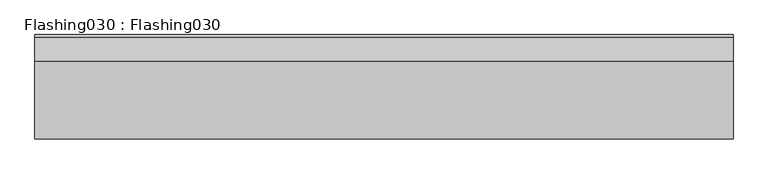
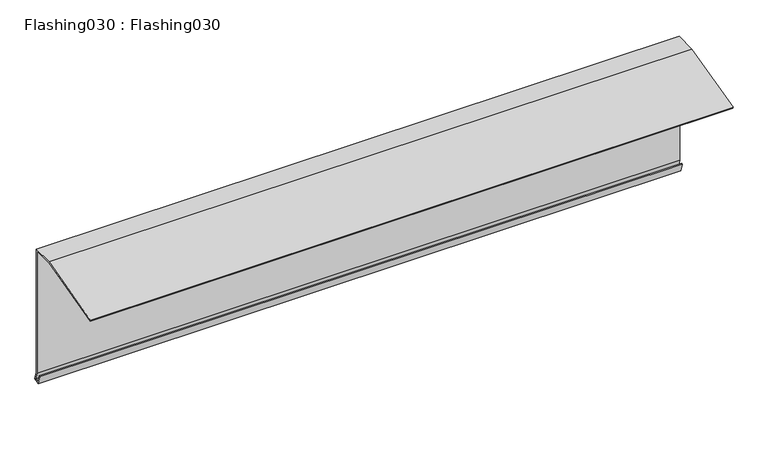
"""IFC4 building model written with IfcOpenShell, lengths in millimetres: proxy geometry, Flashing030 : Flashing030."""

from ifc_helpers import new_model, si_unit, frame, origin, place, context, project, spatial, polyline, outline, extrude, source, transform, mapped, element, save


def flashing030_flashing030_f511b4f4(model_context):
    return source(origin(), model_context, "Body", "SweptSolid", [
        extrude(outline(polyline([(2234.7481762, 44738.1803898), (2303.5709356, 44738.1803898), (2303.5709356, 44333.7602228), (2311.8566846, 44306.7687568), (2294.2946954, 44301.3776367), (2285.7732111, 44328.9010742), (2289.5942634, 44330.0841037), (2296.9371652, 44306.3673555), (2306.8647031, 44309.4000801), (2299.5709356, 44333.1600896), (2299.5709356, 44734.1803898), (2235.2510707, 44734.1803898), (2013.7504579, 44677.5901625), (2012.7603192, 44681.4656787), (2234.7481762, 44738.1803898)])), frame((6470.1466437, 0.0, 0.0), z_axis=(1.0, 0.0, 0.0), x_axis=(0.0, 1.0, 0.0)), (0.0, 0.0, 1.0), 1999.85),
    ])


if __name__ == "__main__":
    model = new_model("IFC4")
    model_context = context("Model", 3, world=origin())
    ifc_project = project(units=[si_unit("LENGTHUNIT", "METRE", prefix="MILLI")], contexts=[model_context])
    site = spatial("IfcSite", under=ifc_project)
    building = spatial("IfcBuilding", under=site)
    placement = place(None, origin())
    flashing030_flashing030_shape = flashing030_flashing030_f511b4f4(model_context)
    element("IfcBuildingElementProxy", 1, Name="Flashing030 : Flashing030", ObjectType="Flashing030 : Flashing030", at=placement, inside=building, context=model_context, shape_type="MappedRepresentation", body=[
        mapped(flashing030_flashing030_shape, transform((0.0, 0.0, 0.0), x_axis=(1.0, 0.0, 0.0), y_axis=(0.0, 1.0, 0.0), z_axis=(0.0, 0.0, 1.0))),
    ])
    save(model, "model.ifc")

# Revit data of these elements
# Type "Flashing030 : Flashing030"
#   NameOverride = "Flashing030"
# Element 1 (IfcBuildingElementProxy, "Flashing030 : Flashing030")
#   Materials on its faces: "BRAKE METAL EAVE TRIM TO MATCH STANDING SEAM COLOR"
# Materials
#   "BRAKE METAL EAVE TRIM TO MATCH STANDING SEAM COLOR": class "Unassigned", colour RGB 128 128 128, transparency 0, Cost = 0
